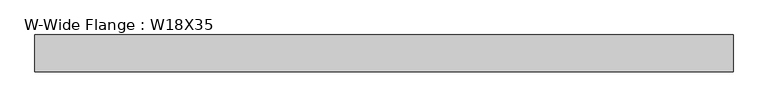
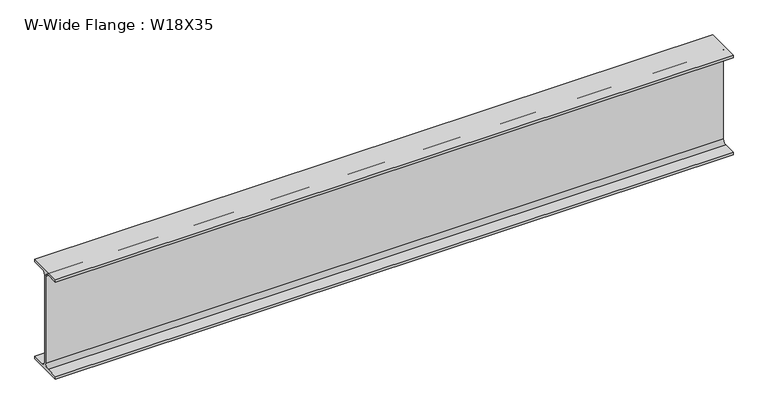
"""IFC4 building model written with IfcOpenShell, lengths in millimetres: beam geometry, W-Wide Flange : W18X35."""

from ifc_helpers import new_model, si_unit, point, frame, frame_2d, origin, place, context, project, spatial, polyline, circle_curve, trimmed, segment, composite_curve, outline, extrude, source, transform, mapped, element, save


def w_wide_flange_w18x35_e843acb2(model_context):
    return source(origin(), model_context, "Body", "SweptSolid", [
        extrude(outline(composite_curve([segment(polyline([(76.2, -213.995), (76.2, -224.79), (-76.2, -224.79), (-76.2, -213.995), (-21.59, -213.995)]), True, "CONTINUOUS"), segment(trimmed(circle_curve(frame_2d((-21.59, -196.215)), 17.78), [point((-21.59, -213.995))], [point((-3.81, -196.215))], True, "CARTESIAN"), True, "CONTINUOUS"), segment(polyline([(-3.81, -196.215), (-3.81, 196.215)]), True, "CONTINUOUS"), segment(trimmed(circle_curve(frame_2d((-21.59, 196.215)), 17.78), [point((-3.81, 196.215))], [point((-21.59, 213.995))], True, "CARTESIAN"), True, "CONTINUOUS"), segment(polyline([(-21.59, 213.995), (-76.2, 213.995), (-76.2, 224.79), (76.2, 224.79), (76.2, 213.995), (21.59, 213.995)]), True, "CONTINUOUS"), segment(trimmed(circle_curve(frame_2d((21.59, 196.215)), 17.78), [point((21.59, 213.995))], [point((3.81, 196.215))], True, "CARTESIAN"), True, "CONTINUOUS"), segment(polyline([(3.81, 196.215), (3.81, -196.215)]), True, "CONTINUOUS"), segment(trimmed(circle_curve(frame_2d((21.59, -196.215)), 17.78), [point((3.81, -196.215))], [point((21.59, -213.995))], True, "CARTESIAN"), True, "CONTINUOUS"), segment(polyline([(21.59, -213.995), (76.2, -213.995)]), True, "CONTINUOUS")], self_intersect=False)), frame((-1424.78125, 0.0, 0.0), z_axis=(1.0, 0.0, 0.0), x_axis=(0.0, 1.0, 0.0)), (0.0, 0.0, 1.0), 2900.3625),
    ])


if __name__ == "__main__":
    model = new_model("IFC4")
    model_context = context("Model", 3, world=origin())
    ifc_project = project(units=[si_unit("LENGTHUNIT", "METRE", prefix="MILLI")], contexts=[model_context])
    site = spatial("IfcSite", under=ifc_project)
    building = spatial("IfcBuilding", under=site)
    placement = place(None, origin())
    w_wide_flange_w18x35_shape = w_wide_flange_w18x35_e843acb2(model_context)
    element("IfcBeam", 1, ObjectType="W-Wide Flange : W18X35", at=placement, inside=building, context=model_context, shape_type="MappedRepresentation", body=[
        mapped(w_wide_flange_w18x35_shape, transform((0.0, 0.0, 0.0), x_axis=(1.0, 0.0, 0.0), y_axis=(0.0, 1.0, 0.0), z_axis=(0.0, 0.0, 1.0))),
    ])
    save(model, "model.ifc")

# Revit data of these elements
# Type "W-Wide Flange : W18X35"
#   Assembly Code = "B10"
#   W = 35
#   Length [instance default] = 5' - 0"
#   bf = 0' - 6"
#   d = 1' - 5.7"
#   k = 0' - 1 1/8"
#   k2 = 0' - 0.7"
#   tf = 0' - 0.425"
#   tw = 0' - 0.3"
#   A = 0.0715278 SF
#   Structural Material [instance default] = Steel ASTM A992
# Element 1 (IfcBeam, "W-Wide Flange : W18X35")
#   Structural Material = Steel ASTM A36
#   Materials on its faces: "Steel ASTM A36"
# Materials
#   "Steel ASTM A992": class "Metal", colour RGB 199 199 199, transparency 0, Description = "Structural steel 50ksi", Cost = 0
#   "Steel ASTM A36": class "Metal", colour RGB 199 199 199, transparency 0, Description = "Structural steel, ASTM A36 Grade B, mill finish", Cost = 0
